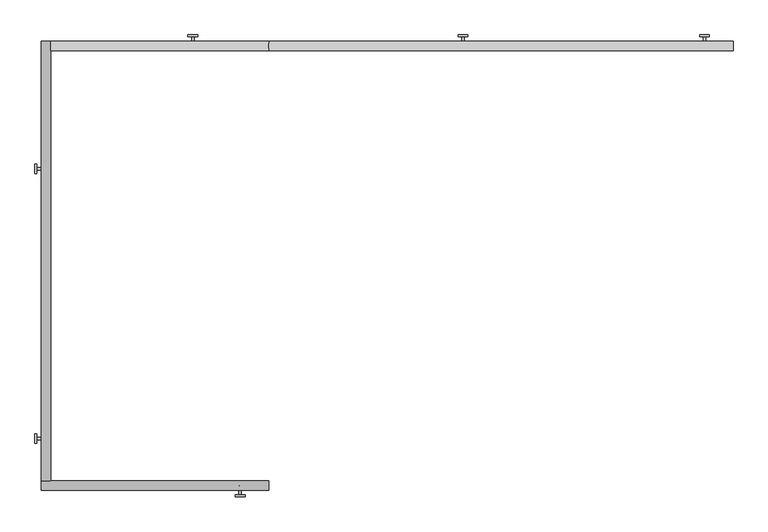
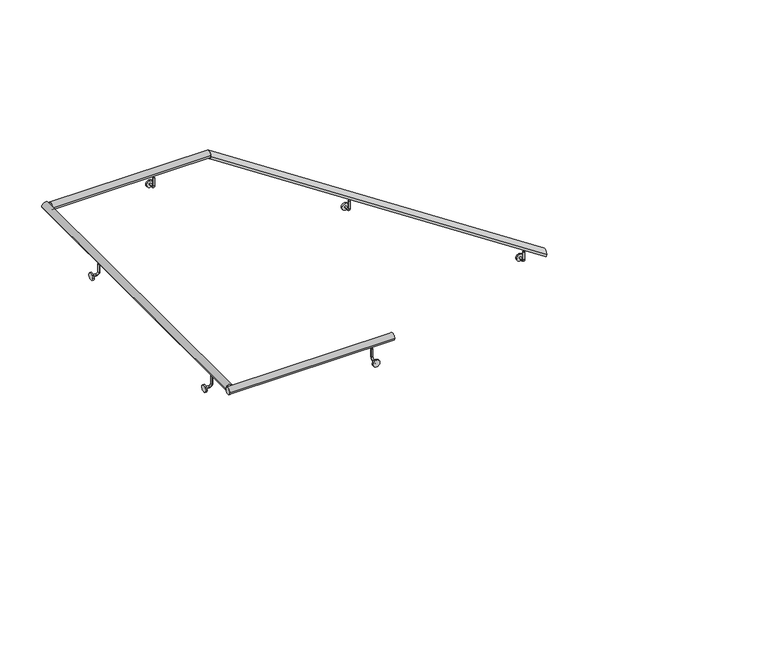
"""IFC4 building model written with IfcOpenShell, lengths in millimetres: railing geometry."""

import ifcopenshell
import ifcopenshell.guid

model = None  # the IFC model being written
_history = None  # IfcOwnerHistory: only IFC2X3 demands one
_inside = {}  # id of a spatial element -> (the spatial element, [elements in it])
_under = {}  # id of a project, library or spatial element -> (it, [spatial elements below it])
_declared = {}  # id of a project -> (the project, [libraries it declares])
_typed = {}  # id of a type object -> (the type object, [elements of that type])
_made_of = {}  # id of a material, layer set ... -> (it, [elements and type objects made of it])


def new_model(schema):
    """Start an empty IFC model of exactly this schema.

    Asked for "IFC4X3", IfcOpenShell would pick the latest addendum, in which some entities
    have other attributes; the version numbers below select the first issue.
    IFC2X3 requires an IfcOwnerHistory on every rooted entity: one is made here for all.
    """
    global model, _history
    if schema == "IFC4X3":
        model = ifcopenshell.file(schema_version=(4, 3, 0, 0))
    else:
        model = ifcopenshell.file(schema=schema)
    _inside.clear()
    _under.clear()
    _declared.clear()
    _typed.clear()
    _made_of.clear()
    _history = None
    if model.schema == "IFC2X3":
        org = make("IfcOrganization", Name="unknown")
        user = make(
            "IfcPersonAndOrganization",
            ThePerson=make("IfcPerson", FamilyName="unknown"),
            TheOrganization=org,
        )
        app = make(
            "IfcApplication",
            ApplicationDeveloper=org,
            Version="unknown",
            ApplicationFullName="unknown",
            ApplicationIdentifier="unknown",
        )
        _history = make(
            "IfcOwnerHistory",
            OwningUser=user,
            OwningApplication=app,
            ChangeAction="ADDED",
            CreationDate=0,
        )
    return model


def make(cls, **values):
    """One entity of the class cls with the attributes given. An attribute that is None is left unset."""
    return model.create_entity(
        cls, **{name: value for name, value in values.items() if value is not None}
    )


def rooted(cls, **values):
    """An entity with a GlobalId (a new one), such as an element, a storey or a relation."""
    return make(cls, GlobalId=ifcopenshell.guid.new(), OwnerHistory=_history, **values)


def si_unit(unit_type, name, prefix=None):
    """IfcSIUnit, for example si_unit("LENGTHUNIT", "METRE", prefix="MILLI")."""
    return make("IfcSIUnit", UnitType=unit_type, Prefix=prefix, Name=name)


def assignment(units):
    """IfcUnitAssignment: the units of a project."""
    return None if units is None else make("IfcUnitAssignment", Units=units)


def point(xyz):
    """IfcCartesianPoint."""
    return None if xyz is None else make("IfcCartesianPoint", Coordinates=xyz)


def direction(xyz):
    """IfcDirection."""
    return None if xyz is None else make("IfcDirection", DirectionRatios=xyz)


def frame(location, z_axis=None, x_axis=None):
    """IfcAxis2Placement3D, a coordinate frame: its origin and axes. An axis left out is left unset."""
    return make(
        "IfcAxis2Placement3D",
        Location=point(location),
        Axis=direction(z_axis),
        RefDirection=direction(x_axis),
    )


def frame_2d(location, x_axis=None):
    """IfcAxis2Placement2D, a coordinate frame in the plane: its origin and x axis."""
    return make(
        "IfcAxis2Placement2D", Location=point(location), RefDirection=direction(x_axis)
    )


def origin():
    """The frame at (0, 0, 0) with its axes left unset."""
    return frame((0.0, 0.0, 0.0))


def place(relative_to, where):
    """IfcLocalPlacement: puts the frame where relative to a parent placement (None: the world)."""
    return make(
        "IfcLocalPlacement", PlacementRelTo=relative_to, RelativePlacement=where
    )


def context(
    kind, dimensions, precision=None, world=None, true_north=None, identifier=None
):
    """IfcGeometricRepresentationContext, for example the 3D "Model" context."""
    return make(
        "IfcGeometricRepresentationContext",
        ContextIdentifier=identifier,
        ContextType=kind,
        CoordinateSpaceDimension=dimensions,
        Precision=precision,
        WorldCoordinateSystem=world,
        TrueNorth=true_north,
    )


def project(units=None, contexts=None):
    """IfcProject with its units and contexts."""
    return rooted(
        "IfcProject",
        Name="project",
        RepresentationContexts=contexts,
        UnitsInContext=assignment(units),
    )


def spatial(cls, under=None, at=None, **own):
    """A site, building, storey or space (cls), placed at a placement, below another one or the project."""
    s = rooted(cls, ObjectPlacement=at, **own)
    if under is not None:
        _under.setdefault(under.id(), (under, []))[1].append(s)
    return s


def circle_curve(where, radius):
    """IfcCircle in the frame where."""
    return make("IfcCircle", Position=where, Radius=radius)


def ellipse_curve(where, semi_axis1, semi_axis2):
    """IfcEllipse in the frame where."""
    return make(
        "IfcEllipse", Position=where, SemiAxis1=semi_axis1, SemiAxis2=semi_axis2
    )


def trimmed(basis, trim1, trim2, sense, master):
    """IfcTrimmedCurve: the piece of a basis curve between two trims."""
    return make(
        "IfcTrimmedCurve",
        BasisCurve=basis,
        Trim1=trim1,
        Trim2=trim2,
        SenseAgreement=sense,
        MasterRepresentation=master,
    )


def segment(curve, same_sense, transition):
    """IfcCompositeCurveSegment."""
    return make(
        "IfcCompositeCurveSegment",
        Transition=transition,
        SameSense=same_sense,
        ParentCurve=curve,
    )


def composite_curve(segments, self_intersect=None):
    """IfcCompositeCurve: segments joined end to end."""
    return make("IfcCompositeCurve", Segments=segments, SelfIntersect=self_intersect)


def outline(outer, holes=None, kind="AREA"):
    """IfcArbitraryClosedProfileDef: a profile drawn as a closed curve; with holes, ...WithVoids."""
    if holes is None:
        return make("IfcArbitraryClosedProfileDef", ProfileType=kind, OuterCurve=outer)
    return make(
        "IfcArbitraryProfileDefWithVoids",
        ProfileType=kind,
        OuterCurve=outer,
        InnerCurves=holes,
    )


def extrude(swept, where, along, depth):
    """IfcExtrudedAreaSolid: the profile swept, set in the frame where, extruded along a direction by depth."""
    return make(
        "IfcExtrudedAreaSolid",
        SweptArea=swept,
        Position=where,
        ExtrudedDirection=direction(along),
        Depth=depth,
    )


def shape(context_of_items, identifier, shape_type, items):
    """IfcShapeRepresentation: the items that make up one representation, for example the "Body"."""
    return make(
        "IfcShapeRepresentation",
        ContextOfItems=context_of_items,
        RepresentationIdentifier=identifier,
        RepresentationType=shape_type,
        Items=items,
    )


def source(mapping_origin, context_of_items, identifier, shape_type, items):
    """IfcRepresentationMap: a shape defined once, which mapped items show again and again."""
    return make(
        "IfcRepresentationMap",
        MappingOrigin=mapping_origin,
        MappedRepresentation=shape(context_of_items, identifier, shape_type, items),
    )


def transform(
    local_origin,
    x_axis=None,
    y_axis=None,
    z_axis=None,
    scale=None,
    scale2=None,
    scale3=None,
    uniform=True,
):
    """IfcCartesianTransformationOperator3D, or its non-uniform kind. x_axis, y_axis, z_axis: its Axis1, 2, 3."""
    if uniform:
        return make(
            "IfcCartesianTransformationOperator3D",
            Axis1=direction(x_axis),
            Axis2=direction(y_axis),
            LocalOrigin=point(local_origin),
            Scale=scale,
            Axis3=direction(z_axis),
        )
    return make(
        "IfcCartesianTransformationOperator3DnonUniform",
        Axis1=direction(x_axis),
        Axis2=direction(y_axis),
        LocalOrigin=point(local_origin),
        Scale=scale,
        Axis3=direction(z_axis),
        Scale2=scale2,
        Scale3=scale3,
    )


def mapped(mapping_source, mapping_target):
    """IfcMappedItem: shows the shape of a source again, moved by a transform."""
    return make(
        "IfcMappedItem", MappingSource=mapping_source, MappingTarget=mapping_target
    )


def made_of(thing, what):
    """Note that an element or type object is made of a material, layer set ...; save() writes the relation."""
    if what is not None:
        _made_of.setdefault(what.id(), (what, []))[1].append(thing)
    return thing


def element(
    cls,
    number,
    at=None,
    inside=None,
    cuts=None,
    type_object=None,
    material=None,
    context=None,
    identifier="Body",
    shape_type=None,
    held_by="IfcProductDefinitionShape",
    body=None,
    shapes=None,
    **own,
):
    """One element of the class cls, such as IfcWall. Its Tag is "e" and its number.

    at: its placement. inside: the storey or other place that contains it. cuts: it is an
    opening in that element (IfcRelVoidsElement). A single representation is given by context,
    identifier, shape_type and body (its items); several are given by shapes. held_by: the class
    of the entity that holds the representations. save() writes the other relations.
    """
    e = rooted(cls, Tag="e%d" % number, ObjectPlacement=at, **own)
    if body is not None:
        shapes = [shape(context, identifier, shape_type, body)]
    if shapes is not None:
        e.Representation = make(held_by, Representations=shapes)
    if inside is not None:
        _inside.setdefault(inside.id(), (inside, []))[1].append(e)
    if cuts is not None:
        rooted(
            "IfcRelVoidsElement", RelatingBuildingElement=cuts, RelatedOpeningElement=e
        )
    if type_object is not None:
        _typed.setdefault(type_object.id(), (type_object, []))[1].append(e)
    return made_of(e, material)


def aggregate(whole, parts):
    """IfcRelAggregates: a whole, such as a stair, and the parts it consists of."""
    return rooted("IfcRelAggregates", RelatingObject=whole, RelatedObjects=parts)


def save(model, path):
    """Write the relations noted so far, then the file.

    IfcRelAggregates (storeys below a building ...), IfcRelContainedInSpatialStructure (elements
    in a storey), IfcRelDefinesByType, IfcRelAssociatesMaterial and IfcRelDeclares: one each for
    every whole, place, type object, material and project.
    """
    for whole, parts in _under.values():
        aggregate(whole, parts)
    for where, things in _inside.values():
        rooted(
            "IfcRelContainedInSpatialStructure",
            RelatedElements=things,
            RelatingStructure=where,
        )
    for kind, things in _typed.values():
        rooted("IfcRelDefinesByType", RelatedObjects=things, RelatingType=kind)
    for what, things in _made_of.values():
        rooted("IfcRelAssociatesMaterial", RelatedObjects=things, RelatingMaterial=what)
    for by, libraries in _declared.values():
        rooted("IfcRelDeclares", RelatingContext=by, RelatedDefinitions=libraries)
    model.write(path)


def plane_surface(at):
    """IfcPlane: the flat surface through the origin of the frame at, square to its z axis."""
    return make("IfcPlane", Position=at)


def cylinder_surface(at, radius):
    """IfcCylindricalSurface: all points at the distance radius from the z axis of the frame at."""
    return make("IfcCylindricalSurface", Position=at, Radius=radius)


def revolved_surface(curve, axis_point, axis_direction):
    """IfcSurfaceOfRevolution: the curve turned about the line through axis_point along axis_direction."""
    return make(
        "IfcSurfaceOfRevolution",
        SweptCurve=make("IfcArbitraryOpenProfileDef", ProfileType="CURVE", Curve=curve),
        AxisPosition=make("IfcAxis1Placement", Location=point(axis_point), Axis=direction(axis_direction)),
    )


def advanced_brep(points, edges, surfaces, faces):
    """IfcAdvancedBrep: a solid bounded by faces that lie on surfaces and meet in shared edges.

    An edge is (start, end): straight between two places in points (the first is 0);
    or (start, end, curve); or (start, end, curve, False) where it runs against its curve.
    A face is (place in surfaces, loops), or (place, loops, False) where it looks against
    its surface's normal. A loop lists edges by number (the first is 1), with a minus sign
    where the edge is run from its end to its start. The first loop is the outer one.
    """
    corners = [point(p) for p in points]
    vertices = [make("IfcVertexPoint", VertexGeometry=c) for c in corners]
    made = []
    for start, end, *more in edges:
        made.append(
            make(
                "IfcEdgeCurve",
                EdgeStart=vertices[start],
                EdgeEnd=vertices[end],
                EdgeGeometry=more[0] if more else make("IfcPolyline", Points=[corners[start], corners[end]]),
                SameSense=more[1] if len(more) > 1 else True,
            )
        )
    hull = []
    for where, loops, *sense in faces:
        bounds = []
        for j, loop in enumerate(loops):
            ring = [make("IfcOrientedEdge", EdgeElement=made[abs(k) - 1], Orientation=k > 0) for k in loop]
            bounds.append(
                make(
                    "IfcFaceOuterBound" if j == 0 else "IfcFaceBound",
                    Bound=make("IfcEdgeLoop", EdgeList=ring),
                    Orientation=True,
                )
            )
        hull.append(make("IfcAdvancedFace", Bounds=bounds, FaceSurface=surfaces[where], SameSense=sense[0] if sense else True))
    return make("IfcAdvancedBrep", Outer=make("IfcClosedShell", CfsFaces=hull))


def railing_2f2e9fd8(model_context):
    return source(origin(), model_context, "Body", "SolidModel", [
        advanced_brep(
        [(-47841.1127262, 17739.1574868, 1147.8451634), (-47841.1127262, 17789.1574868, 1147.8451634), (-50271.1127262, 17739.1574868, 2747.8451634), (-50271.1127262, 17789.1574868, 2747.8451634)],
        [
            (0, 1, ellipse_curve(frame((-47841.1127262, 17764.1574868, 1147.8451634), z_axis=(1.0, 0.0, 0.0), x_axis=(0.0, 0.0, -1.0)), 29.9326144, 25.0)),
            (1, 0, ellipse_curve(frame((-47841.1127262, 17764.1574868, 1147.8451634), z_axis=(1.0, 0.0, 0.0), x_axis=(0.0, 0.0, -1.0)), 29.9326144, 25.0)),
            (2, 3, ellipse_curve(frame((-50271.1127262, 17764.1574868, 2747.8451634), z_axis=(-1.0, 0.0, 0.0), x_axis=(0.0, 0.0, -1.0)), 29.9326144, 25.0)),
            (3, 2, ellipse_curve(frame((-50271.1127262, 17764.1574868, 2747.8451634), z_axis=(-1.0, 0.0, 0.0), x_axis=(0.0, 0.0, -1.0)), 29.9326144, 25.0)),
            (0, 2),
            (3, 1),
        ],
        [
            plane_surface(frame((-47841.1127262, 17764.1574868, 1177.7777778), z_axis=(1.0, 0.0, 0.0), x_axis=(0.0, -1.0, 0.0))),
            plane_surface(frame((-50271.1127262, 17764.1574868, 2777.7777778), z_axis=(-1.0, 0.0, 0.0), x_axis=(0.0, -1.0, 0.0))),
            cylinder_surface(frame((-47854.8610286, 17764.1574868, 1156.8975435), z_axis=(0.8352093694289686, 0.0, -0.5499320950972626), x_axis=(0.0, 1.0, 0.0)), 25.0),
        ],
        [
            (0, [[1, 2]]),
            (1, [[3, 4]]),
            (2, [[-1, 5, -4, 6]]),
            (2, [[-2, -6, -3, -5]]),
        ],
    ),
        advanced_brep(
        [(-50271.1127262, 17739.1574868, 2752.7777778), (-50271.1127262, 17789.1574868, 2752.7777778), (-51413.5127262, 17739.1574868, 2752.7777778), (-51413.5127262, 17789.1574868, 2752.7777778)],
        [
            (0, 1, circle_curve(frame((-50271.1127262, 17764.1574868, 2752.7777778), z_axis=(1.0, 0.0, 0.0), x_axis=(0.0, 1.0, 0.0)), 25.0)),
            (1, 0, circle_curve(frame((-50271.1127262, 17764.1574868, 2752.7777778), z_axis=(1.0, 0.0, 0.0), x_axis=(0.0, 1.0, 0.0)), 25.0)),
            (2, 3, circle_curve(frame((-51413.5127262, 17764.1574868, 2752.7777778), z_axis=(-1.0, 0.0, 0.0), x_axis=(0.0, 1.0, 0.0)), 25.0)),
            (3, 2, circle_curve(frame((-51413.5127262, 17764.1574868, 2752.7777778), z_axis=(-1.0, 0.0, 0.0), x_axis=(0.0, 1.0, 0.0)), 25.0)),
            (0, 2),
            (3, 1),
        ],
        [
            plane_surface(frame((-50271.1127262, 17764.1574868, 2777.7777778), z_axis=(1.0, 0.0, 0.0), x_axis=(0.0, -1.0, 0.0))),
            plane_surface(frame((-51413.5127262, 17764.1574868, 2777.7777778), z_axis=(-1.0, 0.0, 0.0), x_axis=(0.0, -1.0, 0.0))),
            cylinder_surface(frame((-50271.1127262, 17764.1574868, 2752.7777778), z_axis=(1.0, 0.0, 0.0), x_axis=(0.0, 1.0, 0.0)), 25.0),
        ],
        [
            (0, [[1, 2]]),
            (1, [[3, 4]]),
            (2, [[-1, 5, -4, 6]]),
            (2, [[-2, -6, -3, -5]]),
        ],
    ),
        advanced_brep(
        [(-51413.5127262, 17789.1574868, 2752.7777778), (-51463.5127262, 17789.1574868, 2752.7777778), (-51413.5127262, 15484.3587092, 2752.7777778), (-51463.5127262, 15484.3587092, 2752.7777778)],
        [
            (0, 1, circle_curve(frame((-51438.5127262, 17789.1574868, 2752.7777778), z_axis=(0.0, 1.0, 0.0), x_axis=(-1.0, 0.0, 0.0)), 25.0)),
            (1, 0, circle_curve(frame((-51438.5127262, 17789.1574868, 2752.7777778), z_axis=(0.0, 1.0, 0.0), x_axis=(-1.0, 0.0, 0.0)), 25.0)),
            (2, 3, circle_curve(frame((-51438.5127262, 15484.3587092, 2752.7777778), z_axis=(0.0, -1.0, 0.0), x_axis=(-1.0, 0.0, 0.0)), 25.0)),
            (3, 2, circle_curve(frame((-51438.5127262, 15484.3587092, 2752.7777778), z_axis=(0.0, -1.0, 0.0), x_axis=(-1.0, 0.0, 0.0)), 25.0)),
            (0, 2),
            (3, 1),
        ],
        [
            plane_surface(frame((-51438.5127262, 17789.1574868, 2777.7777778), z_axis=(0.0, 1.0, 0.0), x_axis=(0.0, 0.0, -1.0))),
            plane_surface(frame((-51438.5127262, 15484.3587092, 2777.7777778), z_axis=(0.0, -1.0, 0.0), x_axis=(0.0, 0.0, -1.0))),
            cylinder_surface(frame((-51438.5127262, 17789.1574868, 2752.7777778), z_axis=(0.0, 1.0, 0.0), x_axis=(-1.0, 0.0, 0.0)), 25.0),
        ],
        [
            (0, [[1, 2]]),
            (1, [[3, 4]]),
            (2, [[-1, 5, -4, 6]]),
            (2, [[-2, -6, -3, -5]]),
        ],
    ),
        advanced_brep(
        [(-51463.5127262, 15484.3587092, 2752.7777778), (-51463.5127262, 15434.3587092, 2752.7777778), (-50271.1127262, 15484.3587092, 2752.7777778), (-50271.1127262, 15434.3587092, 2752.7777778)],
        [
            (0, 1, circle_curve(frame((-51463.5127262, 15459.3587092, 2752.7777778), z_axis=(-1.0, 0.0, 0.0), x_axis=(0.0, -1.0, 0.0)), 25.0)),
            (1, 0, circle_curve(frame((-51463.5127262, 15459.3587092, 2752.7777778), z_axis=(-1.0, 0.0, 0.0), x_axis=(0.0, -1.0, 0.0)), 25.0)),
            (2, 3, circle_curve(frame((-50271.1127262, 15459.3587092, 2752.7777778), z_axis=(1.0, 0.0, 0.0), x_axis=(0.0, -1.0, 0.0)), 25.0)),
            (3, 2, circle_curve(frame((-50271.1127262, 15459.3587092, 2752.7777778), z_axis=(1.0, 0.0, 0.0), x_axis=(0.0, -1.0, 0.0)), 25.0)),
            (0, 2),
            (3, 1),
        ],
        [
            plane_surface(frame((-51463.5127262, 15459.3587092, 2777.7777778), z_axis=(-1.0, 0.0, 0.0), x_axis=(0.0, 1.0, 0.0))),
            plane_surface(frame((-50271.1127262, 15459.3587092, 2777.7777778), z_axis=(1.0, 0.0, 0.0), x_axis=(0.0, 1.0, 0.0))),
            cylinder_surface(frame((-51463.5127262, 15459.3587092, 2752.7777778), z_axis=(-1.0, 0.0, 0.0), x_axis=(0.0, -1.0, 0.0)), 25.0),
        ],
        [
            (0, [[1, 2]]),
            (1, [[3, 4]]),
            (2, [[-1, 5, -4, 6]]),
            (2, [[-2, -6, -3, -5]]),
        ],
    ),
        advanced_brep(
        [(-51438.5127262, 15712.2284647, 2708.7277778), (-51438.5127262, 15699.5284647, 2708.7277778), (-51438.5127262, 15712.2284647, 2651.5777778), (-51438.5127262, 15699.5284647, 2651.5777778), (-51457.5627262, 15699.5284647, 2632.5277778), (-51457.5627262, 15712.2284647, 2632.5277778), (-51486.1377262, 15712.2284647, 2632.5277778), (-51486.1377262, 15699.5284647, 2632.5277778)],
        [
            (0, 1, circle_curve(frame((-51438.5127262, 15705.8784647, 2708.7277778), z_axis=(0.0, 0.0, 1.0), x_axis=(0.0, -1.0, 0.0)), 6.35)),
            (1, 0, circle_curve(frame((-51438.5127262, 15705.8784647, 2708.7277778), z_axis=(0.0, 0.0, 1.0), x_axis=(0.0, -1.0, 0.0)), 6.35)),
            (0, 2),
            (2, 3, circle_curve(frame((-51438.5127262, 15705.8784647, 2651.5777778), z_axis=(0.0, 0.0, 1.0), x_axis=(0.0, -1.0, 0.0)), 6.35)),
            (3, 1),
            (3, 2, circle_curve(frame((-51438.5127262, 15705.8784647, 2651.5777778), z_axis=(0.0, 0.0, 1.0), x_axis=(0.0, -1.0, 0.0)), 6.35)),
            (4, 3, circle_curve(frame((-51457.5627262, 15699.5284647, 2651.5777778), z_axis=(0.0, -1.0, 0.0), x_axis=(1.0, 0.0, 0.0)), 19.05)),
            (2, 5, circle_curve(frame((-51457.5627262, 15712.2284647, 2651.5777778), z_axis=(0.0, 1.0, 0.0), x_axis=(1.0, 0.0, 0.0)), 19.05)),
            (5, 4, circle_curve(frame((-51457.5627262, 15705.8784647, 2632.5277778), z_axis=(1.0, 0.0, 0.0), x_axis=(0.0, -1.0, 0.0)), 6.35)),
            (4, 5, circle_curve(frame((-51457.5627262, 15705.8784647, 2632.5277778), z_axis=(1.0, 0.0, 0.0), x_axis=(0.0, -1.0, 0.0)), 6.35)),
            (6, 7, circle_curve(frame((-51486.1377262, 15705.8784647, 2632.5277778), z_axis=(-1.0, 0.0, 0.0), x_axis=(0.0, -1.0, 0.0)), 6.35)),
            (7, 6, circle_curve(frame((-51486.1377262, 15705.8784647, 2632.5277778), z_axis=(-1.0, 0.0, 0.0), x_axis=(0.0, -1.0, 0.0)), 6.35)),
            (5, 6),
            (7, 4),
        ],
        [
            plane_surface(frame((-51438.5127262, 15699.5284647, 2708.7277778), z_axis=(0.0, 0.0, 1.0), x_axis=(-1.0, 0.0, 0.0))),
            cylinder_surface(frame((-51438.5127262, 15705.8784647, 2708.7277778), z_axis=(0.0, 0.0, 1.0), x_axis=(0.0, -1.0, 0.0)), 6.35),
            revolved_surface(trimmed(ellipse_curve(frame((-51438.5127262, 15705.8784647, 2651.5777778), z_axis=(0.0, 0.0, 1.0), x_axis=(0.0, -1.0, 0.0)), 6.35, 6.35), [point((-51438.5127262, 15712.2284647, 2651.5777778))], [point((-51438.5127262, 15699.5284647, 2651.5777778))], True, "CARTESIAN"), (-51457.5627262, 15705.8784647, 2651.5777778), (0.0, 1.0, 0.0)),
            revolved_surface(trimmed(ellipse_curve(frame((-51438.5127262, 15705.8784647, 2651.5777778), z_axis=(0.0, 0.0, 1.0), x_axis=(0.0, -1.0, 0.0)), 6.35, 6.35), [point((-51438.5127262, 15699.5284647, 2651.5777778))], [point((-51438.5127262, 15712.2284647, 2651.5777778))], True, "CARTESIAN"), (-51457.5627262, 15705.8784647, 2651.5777778), (0.0, 1.0, 0.0)),
            plane_surface(frame((-51486.1377262, 15705.8784647, 2626.1777778), z_axis=(-1.0, 0.0, 0.0), x_axis=(0.0, -1.0, 0.0))),
            cylinder_surface(frame((-51457.5627262, 15705.8784647, 2632.5277778), z_axis=(1.0, 0.0, 0.0), x_axis=(0.0, -1.0, 0.0)), 6.35),
        ],
        [
            (0, [[1, 2]]),
            (1, [[-1, 3, 4, 5]]),
            (1, [[-2, -5, 6, -3]]),
            (2, [[7, -4, 8, 9]]),
            (3, [[-8, -6, -7, 10]]),
            (4, [[11, 12]]),
            (5, [[-9, 13, -12, 14]]),
            (5, [[-10, -14, -11, -13]]),
        ],
    ),
        extrude(outline(composite_curve([segment(trimmed(circle_curve(frame_2d((15705.8784647, 2632.5277778)), 25.4), [point((15680.4784647, 2632.5277778))], [point((15731.2784647, 2632.5277778))], False, "CARTESIAN"), True, "CONTINUOUS"), segment(trimmed(circle_curve(frame_2d((15705.8784647, 2632.5277778)), 25.4), [point((15731.2784647, 2632.5277778))], [point((15680.4784647, 2632.5277778))], False, "CARTESIAN"), True, "CONTINUOUS")], self_intersect=False)), frame((-51495.6627262, 0.0, 0.0), z_axis=(1.0, 0.0, 0.0), x_axis=(0.0, 1.0, 0.0)), (0.0, 0.0, 1.0), 9.525),
        advanced_brep(
        [(-51438.5127262, 17126.1482202, 2708.7277778), (-51438.5127262, 17113.4482202, 2708.7277778), (-51438.5127262, 17126.1482202, 2651.5777778), (-51438.5127262, 17113.4482202, 2651.5777778), (-51457.5627262, 17113.4482202, 2632.5277778), (-51457.5627262, 17126.1482202, 2632.5277778), (-51486.1377262, 17126.1482202, 2632.5277778), (-51486.1377262, 17113.4482202, 2632.5277778)],
        [
            (0, 1, circle_curve(frame((-51438.5127262, 17119.7982202, 2708.7277778), z_axis=(0.0, 0.0, 1.0), x_axis=(0.0, -1.0, 0.0)), 6.35)),
            (1, 0, circle_curve(frame((-51438.5127262, 17119.7982202, 2708.7277778), z_axis=(0.0, 0.0, 1.0), x_axis=(0.0, -1.0, 0.0)), 6.35)),
            (0, 2),
            (2, 3, circle_curve(frame((-51438.5127262, 17119.7982202, 2651.5777778), z_axis=(0.0, 0.0, 1.0), x_axis=(0.0, -1.0, 0.0)), 6.35)),
            (3, 1),
            (3, 2, circle_curve(frame((-51438.5127262, 17119.7982202, 2651.5777778), z_axis=(0.0, 0.0, 1.0), x_axis=(0.0, -1.0, 0.0)), 6.35)),
            (4, 3, circle_curve(frame((-51457.5627262, 17113.4482202, 2651.5777778), z_axis=(0.0, -1.0, 0.0), x_axis=(1.0, 0.0, 0.0)), 19.05)),
            (2, 5, circle_curve(frame((-51457.5627262, 17126.1482202, 2651.5777778), z_axis=(0.0, 1.0, 0.0), x_axis=(1.0, 0.0, 0.0)), 19.05)),
            (5, 4, circle_curve(frame((-51457.5627262, 17119.7982202, 2632.5277778), z_axis=(1.0, 0.0, 0.0), x_axis=(0.0, -1.0, 0.0)), 6.35)),
            (4, 5, circle_curve(frame((-51457.5627262, 17119.7982202, 2632.5277778), z_axis=(1.0, 0.0, 0.0), x_axis=(0.0, -1.0, 0.0)), 6.35)),
            (6, 7, circle_curve(frame((-51486.1377262, 17119.7982202, 2632.5277778), z_axis=(-1.0, 0.0, 0.0), x_axis=(0.0, -1.0, 0.0)), 6.35)),
            (7, 6, circle_curve(frame((-51486.1377262, 17119.7982202, 2632.5277778), z_axis=(-1.0, 0.0, 0.0), x_axis=(0.0, -1.0, 0.0)), 6.35)),
            (5, 6),
            (7, 4),
        ],
        [
            plane_surface(frame((-51438.5127262, 17113.4482202, 2708.7277778), z_axis=(0.0, 0.0, 1.0), x_axis=(-1.0, 0.0, 0.0))),
            cylinder_surface(frame((-51438.5127262, 17119.7982202, 2708.7277778), z_axis=(0.0, 0.0, 1.0), x_axis=(0.0, -1.0, 0.0)), 6.35),
            revolved_surface(trimmed(ellipse_curve(frame((-51438.5127262, 17119.7982202, 2651.5777778), z_axis=(0.0, 0.0, 1.0), x_axis=(0.0, -1.0, 0.0)), 6.35, 6.35), [point((-51438.5127262, 17126.1482202, 2651.5777778))], [point((-51438.5127262, 17113.4482202, 2651.5777778))], True, "CARTESIAN"), (-51457.5627262, 17119.7982202, 2651.5777778), (0.0, 1.0, 0.0)),
            revolved_surface(trimmed(ellipse_curve(frame((-51438.5127262, 17119.7982202, 2651.5777778), z_axis=(0.0, 0.0, 1.0), x_axis=(0.0, -1.0, 0.0)), 6.35, 6.35), [point((-51438.5127262, 17113.4482202, 2651.5777778))], [point((-51438.5127262, 17126.1482202, 2651.5777778))], True, "CARTESIAN"), (-51457.5627262, 17119.7982202, 2651.5777778), (0.0, 1.0, 0.0)),
            plane_surface(frame((-51486.1377262, 17119.7982202, 2626.1777778), z_axis=(-1.0, 0.0, 0.0), x_axis=(0.0, -1.0, 0.0))),
            cylinder_surface(frame((-51457.5627262, 17119.7982202, 2632.5277778), z_axis=(1.0, 0.0, 0.0), x_axis=(0.0, -1.0, 0.0)), 6.35),
        ],
        [
            (0, [[1, 2]]),
            (1, [[-1, 3, 4, 5]]),
            (1, [[-2, -5, 6, -3]]),
            (2, [[7, -4, 8, 9]]),
            (3, [[-8, -6, -7, 10]]),
            (4, [[11, 12]]),
            (5, [[-9, 13, -12, 14]]),
            (5, [[-10, -14, -11, -13]]),
        ],
    ),
        extrude(outline(composite_curve([segment(trimmed(circle_curve(frame_2d((17119.7982202, 2632.5277778)), 25.4), [point((17094.3982202, 2632.5277778))], [point((17145.1982202, 2632.5277778))], False, "CARTESIAN"), True, "CONTINUOUS"), segment(trimmed(circle_curve(frame_2d((17119.7982202, 2632.5277778)), 25.4), [point((17145.1982202, 2632.5277778))], [point((17094.3982202, 2632.5277778))], False, "CARTESIAN"), True, "CONTINUOUS")], self_intersect=False)), frame((-51495.6627262, 0.0, 0.0), z_axis=(1.0, 0.0, 0.0), x_axis=(0.0, 1.0, 0.0)), (0.0, 0.0, 1.0), 9.525),
        advanced_brep(
        [(-50662.6022373, 17764.1574868, 2708.7277778), (-50675.3022373, 17764.1574868, 2708.7277778), (-50662.6022373, 17764.1574868, 2651.5777778), (-50675.3022373, 17764.1574868, 2651.5777778), (-50675.3022373, 17783.2074868, 2632.5277778), (-50662.6022373, 17783.2074868, 2632.5277778), (-50662.6022373, 17811.7824868, 2632.5277778), (-50675.3022373, 17811.7824868, 2632.5277778)],
        [
            (0, 1, circle_curve(frame((-50668.9522373, 17764.1574868, 2708.7277778), z_axis=(0.0, 0.0, 1.0), x_axis=(-1.0, 0.0, 0.0)), 6.35)),
            (1, 0, circle_curve(frame((-50668.9522373, 17764.1574868, 2708.7277778), z_axis=(0.0, 0.0, 1.0), x_axis=(-1.0, 0.0, 0.0)), 6.35)),
            (0, 2),
            (2, 3, circle_curve(frame((-50668.9522373, 17764.1574868, 2651.5777778), z_axis=(0.0, 0.0, 1.0), x_axis=(-1.0, 0.0, 0.0)), 6.35)),
            (3, 1),
            (3, 2, circle_curve(frame((-50668.9522373, 17764.1574868, 2651.5777778), z_axis=(0.0, 0.0, 1.0), x_axis=(-1.0, 0.0, 0.0)), 6.35)),
            (4, 3, circle_curve(frame((-50675.3022373, 17783.2074868, 2651.5777778), z_axis=(-1.0, 0.0, 0.0), x_axis=(0.0, -1.0, 0.0)), 19.05)),
            (2, 5, circle_curve(frame((-50662.6022373, 17783.2074868, 2651.5777778), z_axis=(1.0, 0.0, 0.0), x_axis=(0.0, -1.0, 0.0)), 19.05)),
            (5, 4, circle_curve(frame((-50668.9522373, 17783.2074868, 2632.5277778), z_axis=(0.0, -1.0, 0.0), x_axis=(-1.0, 0.0, 0.0)), 6.35)),
            (4, 5, circle_curve(frame((-50668.9522373, 17783.2074868, 2632.5277778), z_axis=(0.0, -1.0, 0.0), x_axis=(-1.0, 0.0, 0.0)), 6.35)),
            (6, 7, circle_curve(frame((-50668.9522373, 17811.7824868, 2632.5277778), z_axis=(0.0, 1.0, 0.0), x_axis=(-1.0, 0.0, 0.0)), 6.35)),
            (7, 6, circle_curve(frame((-50668.9522373, 17811.7824868, 2632.5277778), z_axis=(0.0, 1.0, 0.0), x_axis=(-1.0, 0.0, 0.0)), 6.35)),
            (5, 6),
            (7, 4),
        ],
        [
            plane_surface(frame((-50675.3022373, 17764.1574868, 2708.7277778), z_axis=(0.0, 0.0, 1.0), x_axis=(0.0, 1.0, 0.0))),
            cylinder_surface(frame((-50668.9522373, 17764.1574868, 2708.7277778), z_axis=(0.0, 0.0, 1.0), x_axis=(-1.0, 0.0, 0.0)), 6.35),
            revolved_surface(trimmed(ellipse_curve(frame((-50668.9522373, 17764.1574868, 2651.5777778), z_axis=(0.0, 0.0, 1.0), x_axis=(-1.0, 0.0, 0.0)), 6.35, 6.35), [point((-50662.6022373, 17764.1574868, 2651.5777778))], [point((-50675.3022373, 17764.1574868, 2651.5777778))], True, "CARTESIAN"), (-50668.9522373, 17783.2074868, 2651.5777778), (1.0, 0.0, 0.0)),
            revolved_surface(trimmed(ellipse_curve(frame((-50668.9522373, 17764.1574868, 2651.5777778), z_axis=(0.0, 0.0, 1.0), x_axis=(-1.0, 0.0, 0.0)), 6.35, 6.35), [point((-50675.3022373, 17764.1574868, 2651.5777778))], [point((-50662.6022373, 17764.1574868, 2651.5777778))], True, "CARTESIAN"), (-50668.9522373, 17783.2074868, 2651.5777778), (1.0, 0.0, 0.0)),
            plane_surface(frame((-50668.9522373, 17811.7824868, 2626.1777778), z_axis=(0.0, 1.0, 0.0), x_axis=(-1.0, 0.0, 0.0))),
            cylinder_surface(frame((-50668.9522373, 17783.2074868, 2632.5277778), z_axis=(0.0, -1.0, 0.0), x_axis=(-1.0, 0.0, 0.0)), 6.35),
        ],
        [
            (0, [[1, 2]]),
            (1, [[-1, 3, 4, 5]]),
            (1, [[-2, -5, 6, -3]]),
            (2, [[7, -4, 8, 9]]),
            (3, [[-8, -6, -7, 10]]),
            (4, [[11, 12]]),
            (5, [[-9, 13, -12, 14]]),
            (5, [[-10, -14, -11, -13]]),
        ],
    ),
        extrude(outline(composite_curve([segment(trimmed(circle_curve(frame_2d((2632.5277778, -50668.9522373)), 25.4), [point((2632.5277778, -50694.3522373))], [point((2632.5277778, -50643.5522373))], False, "CARTESIAN"), True, "CONTINUOUS"), segment(trimmed(circle_curve(frame_2d((2632.5277778, -50668.9522373)), 25.4), [point((2632.5277778, -50643.5522373))], [point((2632.5277778, -50694.3522373))], False, "CARTESIAN"), True, "CONTINUOUS")], self_intersect=False)), frame((0.0, 17811.7824868, 0.0), z_axis=(0.0, 1.0, 0.0), x_axis=(0.0, 0.0, 1.0)), (0.0, 0.0, 1.0), 9.525),
        advanced_brep(
        [(-49248.6824817, 17764.1574868, 2039.7037485), (-49261.3824817, 17764.1574868, 2039.7037485), (-49248.6824817, 17764.1574868, 1982.5537485), (-49261.3824817, 17764.1574868, 1982.5537485), (-49261.3824817, 17783.2074868, 1963.5037485), (-49248.6824817, 17783.2074868, 1963.5037485), (-49248.6824817, 17811.7824868, 1963.5037485), (-49261.3824817, 17811.7824868, 1963.5037485)],
        [
            (0, 1, circle_curve(frame((-49255.0324817, 17764.1574868, 2039.7037485), z_axis=(0.0, 0.0, 1.0), x_axis=(-1.0, 0.0, 0.0)), 6.35)),
            (1, 0, circle_curve(frame((-49255.0324817, 17764.1574868, 2039.7037485), z_axis=(0.0, 0.0, 1.0), x_axis=(-1.0, 0.0, 0.0)), 6.35)),
            (0, 2),
            (2, 3, circle_curve(frame((-49255.0324817, 17764.1574868, 1982.5537485), z_axis=(0.0, 0.0, 1.0), x_axis=(-1.0, 0.0, 0.0)), 6.35)),
            (3, 1),
            (3, 2, circle_curve(frame((-49255.0324817, 17764.1574868, 1982.5537485), z_axis=(0.0, 0.0, 1.0), x_axis=(-1.0, 0.0, 0.0)), 6.35)),
            (4, 3, circle_curve(frame((-49261.3824817, 17783.2074868, 1982.5537485), z_axis=(-1.0, 0.0, 0.0), x_axis=(0.0, -1.0, 0.0)), 19.05)),
            (2, 5, circle_curve(frame((-49248.6824817, 17783.2074868, 1982.5537485), z_axis=(1.0, 0.0, 0.0), x_axis=(0.0, -1.0, 0.0)), 19.05)),
            (5, 4, circle_curve(frame((-49255.0324817, 17783.2074868, 1963.5037485), z_axis=(0.0, -1.0, 0.0), x_axis=(-1.0, 0.0, 0.0)), 6.35)),
            (4, 5, circle_curve(frame((-49255.0324817, 17783.2074868, 1963.5037485), z_axis=(0.0, -1.0, 0.0), x_axis=(-1.0, 0.0, 0.0)), 6.35)),
            (6, 7, circle_curve(frame((-49255.0324817, 17811.7824868, 1963.5037485), z_axis=(0.0, 1.0, 0.0), x_axis=(-1.0, 0.0, 0.0)), 6.35)),
            (7, 6, circle_curve(frame((-49255.0324817, 17811.7824868, 1963.5037485), z_axis=(0.0, 1.0, 0.0), x_axis=(-1.0, 0.0, 0.0)), 6.35)),
            (5, 6),
            (7, 4),
        ],
        [
            plane_surface(frame((-49261.3824817, 17764.1574868, 2039.7037485), z_axis=(0.0, 0.0, 1.0), x_axis=(0.0, 1.0, 0.0))),
            cylinder_surface(frame((-49255.0324817, 17764.1574868, 2039.7037485), z_axis=(0.0, 0.0, 1.0), x_axis=(-1.0, 0.0, 0.0)), 6.35),
            revolved_surface(trimmed(ellipse_curve(frame((-49255.0324817, 17764.1574868, 1982.5537485), z_axis=(0.0, 0.0, 1.0), x_axis=(-1.0, 0.0, 0.0)), 6.35, 6.35), [point((-49248.6824817, 17764.1574868, 1982.5537485))], [point((-49261.3824817, 17764.1574868, 1982.5537485))], True, "CARTESIAN"), (-49255.0324817, 17783.2074868, 1982.5537485), (1.0, 0.0, 0.0)),
            revolved_surface(trimmed(ellipse_curve(frame((-49255.0324817, 17764.1574868, 1982.5537485), z_axis=(0.0, 0.0, 1.0), x_axis=(-1.0, 0.0, 0.0)), 6.35, 6.35), [point((-49261.3824817, 17764.1574868, 1982.5537485))], [point((-49248.6824817, 17764.1574868, 1982.5537485))], True, "CARTESIAN"), (-49255.0324817, 17783.2074868, 1982.5537485), (1.0, 0.0, 0.0)),
            plane_surface(frame((-49255.0324817, 17811.7824868, 1957.1537485), z_axis=(0.0, 1.0, 0.0), x_axis=(-1.0, 0.0, 0.0))),
            cylinder_surface(frame((-49255.0324817, 17783.2074868, 1963.5037485), z_axis=(0.0, -1.0, 0.0), x_axis=(-1.0, 0.0, 0.0)), 6.35),
        ],
        [
            (0, [[1, 2]]),
            (1, [[-1, 3, 4, 5]]),
            (1, [[-2, -5, 6, -3]]),
            (2, [[7, -4, 8, 9]]),
            (3, [[-8, -6, -7, 10]]),
            (4, [[11, 12]]),
            (5, [[-9, 13, -12, 14]]),
            (5, [[-10, -14, -11, -13]]),
        ],
    ),
        extrude(outline(composite_curve([segment(trimmed(circle_curve(frame_2d((1963.5037485, -49255.0324817)), 25.4), [point((1963.5037485, -49280.4324817))], [point((1963.5037485, -49229.6324817))], False, "CARTESIAN"), True, "CONTINUOUS"), segment(trimmed(circle_curve(frame_2d((1963.5037485, -49255.0324817)), 25.4), [point((1963.5037485, -49229.6324817))], [point((1963.5037485, -49280.4324817))], False, "CARTESIAN"), True, "CONTINUOUS")], self_intersect=False)), frame((0.0, 17811.7824868, 0.0), z_axis=(0.0, 1.0, 0.0), x_axis=(0.0, 0.0, 1.0)), (0.0, 0.0, 1.0), 9.525),
        advanced_brep(
        [(-50427.4627262, 15459.3587092, 2708.7277778), (-50414.7627262, 15459.3587092, 2708.7277778), (-50427.4627262, 15459.3587092, 2651.5777778), (-50414.7627262, 15459.3587092, 2651.5777778), (-50414.7627262, 15440.3087092, 2632.5277778), (-50427.4627262, 15440.3087092, 2632.5277778), (-50427.4627262, 15411.7337092, 2632.5277778), (-50414.7627262, 15411.7337092, 2632.5277778)],
        [
            (0, 1, circle_curve(frame((-50421.1127262, 15459.3587092, 2708.7277778), z_axis=(0.0, 0.0, 1.0), x_axis=(1.0, 0.0, 0.0)), 6.35)),
            (1, 0, circle_curve(frame((-50421.1127262, 15459.3587092, 2708.7277778), z_axis=(0.0, 0.0, 1.0), x_axis=(1.0, 0.0, 0.0)), 6.35)),
            (0, 2),
            (2, 3, circle_curve(frame((-50421.1127262, 15459.3587092, 2651.5777778), z_axis=(0.0, 0.0, 1.0), x_axis=(1.0, 0.0, 0.0)), 6.35)),
            (3, 1),
            (3, 2, circle_curve(frame((-50421.1127262, 15459.3587092, 2651.5777778), z_axis=(0.0, 0.0, 1.0), x_axis=(1.0, 0.0, 0.0)), 6.35)),
            (4, 3, circle_curve(frame((-50414.7627262, 15440.3087092, 2651.5777778), z_axis=(1.0, 0.0, 0.0), x_axis=(0.0, 1.0, 0.0)), 19.05)),
            (2, 5, circle_curve(frame((-50427.4627262, 15440.3087092, 2651.5777778), z_axis=(-1.0, 0.0, 0.0), x_axis=(0.0, 1.0, 0.0)), 19.05)),
            (5, 4, circle_curve(frame((-50421.1127262, 15440.3087092, 2632.5277778), z_axis=(0.0, 1.0, 0.0), x_axis=(1.0, 0.0, 0.0)), 6.35)),
            (4, 5, circle_curve(frame((-50421.1127262, 15440.3087092, 2632.5277778), z_axis=(0.0, 1.0, 0.0), x_axis=(1.0, 0.0, 0.0)), 6.35)),
            (6, 7, circle_curve(frame((-50421.1127262, 15411.7337092, 2632.5277778), z_axis=(0.0, -1.0, 0.0), x_axis=(1.0, 0.0, 0.0)), 6.35)),
            (7, 6, circle_curve(frame((-50421.1127262, 15411.7337092, 2632.5277778), z_axis=(0.0, -1.0, 0.0), x_axis=(1.0, 0.0, 0.0)), 6.35)),
            (5, 6),
            (7, 4),
        ],
        [
            plane_surface(frame((-50414.7627262, 15459.3587092, 2708.7277778), z_axis=(0.0, 0.0, 1.0), x_axis=(0.0, -1.0, 0.0))),
            cylinder_surface(frame((-50421.1127262, 15459.3587092, 2708.7277778), z_axis=(0.0, 0.0, 1.0), x_axis=(1.0, 0.0, 0.0)), 6.35),
            revolved_surface(trimmed(ellipse_curve(frame((-50421.1127262, 15459.3587092, 2651.5777778), z_axis=(0.0, 0.0, 1.0), x_axis=(1.0, 0.0, 0.0)), 6.35, 6.35), [point((-50427.4627262, 15459.3587092, 2651.5777778))], [point((-50414.7627262, 15459.3587092, 2651.5777778))], True, "CARTESIAN"), (-50421.1127262, 15440.3087092, 2651.5777778), (-1.0, 0.0, 0.0)),
            revolved_surface(trimmed(ellipse_curve(frame((-50421.1127262, 15459.3587092, 2651.5777778), z_axis=(0.0, 0.0, 1.0), x_axis=(1.0, 0.0, 0.0)), 6.35, 6.35), [point((-50414.7627262, 15459.3587092, 2651.5777778))], [point((-50427.4627262, 15459.3587092, 2651.5777778))], True, "CARTESIAN"), (-50421.1127262, 15440.3087092, 2651.5777778), (-1.0, 0.0, 0.0)),
            plane_surface(frame((-50421.1127262, 15411.7337092, 2626.1777778), z_axis=(0.0, -1.0, 0.0), x_axis=(1.0, 0.0, 0.0))),
            cylinder_surface(frame((-50421.1127262, 15440.3087092, 2632.5277778), z_axis=(0.0, 1.0, 0.0), x_axis=(1.0, 0.0, 0.0)), 6.35),
        ],
        [
            (0, [[1, 2]]),
            (1, [[-1, 3, 4, 5]]),
            (1, [[-2, -5, 6, -3]]),
            (2, [[7, -4, 8, 9]]),
            (3, [[-8, -6, -7, 10]]),
            (4, [[11, 12]]),
            (5, [[-9, 13, -12, 14]]),
            (5, [[-10, -14, -11, -13]]),
        ],
    ),
        extrude(outline(composite_curve([segment(trimmed(circle_curve(frame_2d((2632.5277778, -50421.1127262)), 25.4), [point((2632.5277778, -50395.7127262))], [point((2632.5277778, -50446.5127262))], False, "CARTESIAN"), True, "CONTINUOUS"), segment(trimmed(circle_curve(frame_2d((2632.5277778, -50421.1127262)), 25.4), [point((2632.5277778, -50446.5127262))], [point((2632.5277778, -50395.7127262))], False, "CARTESIAN"), True, "CONTINUOUS")], self_intersect=False)), frame((0.0, 15402.2087092, 0.0), z_axis=(0.0, 1.0, 0.0), x_axis=(0.0, 0.0, 1.0)), (0.0, 0.0, 1.0), 9.525),
        advanced_brep(
        [(-47984.7627262, 17764.1574868, 1207.4932099), (-47997.4627262, 17764.1574868, 1207.4932099), (-47984.7627262, 17764.1574868, 1150.3432099), (-47997.4627262, 17764.1574868, 1150.3432099), (-47997.4627262, 17783.2074868, 1131.2932099), (-47984.7627262, 17783.2074868, 1131.2932099), (-47984.7627262, 17811.7824868, 1131.2932099), (-47997.4627262, 17811.7824868, 1131.2932099)],
        [
            (0, 1, circle_curve(frame((-47991.1127262, 17764.1574868, 1207.4932099), z_axis=(0.0, 0.0, 1.0), x_axis=(-1.0, 0.0, 0.0)), 6.35)),
            (1, 0, circle_curve(frame((-47991.1127262, 17764.1574868, 1207.4932099), z_axis=(0.0, 0.0, 1.0), x_axis=(-1.0, 0.0, 0.0)), 6.35)),
            (0, 2),
            (2, 3, circle_curve(frame((-47991.1127262, 17764.1574868, 1150.3432099), z_axis=(0.0, 0.0, 1.0), x_axis=(-1.0, 0.0, 0.0)), 6.35)),
            (3, 1),
            (3, 2, circle_curve(frame((-47991.1127262, 17764.1574868, 1150.3432099), z_axis=(0.0, 0.0, 1.0), x_axis=(-1.0, 0.0, 0.0)), 6.35)),
            (4, 3, circle_curve(frame((-47997.4627262, 17783.2074868, 1150.3432099), z_axis=(-1.0, 0.0, 0.0), x_axis=(0.0, -1.0, 0.0)), 19.05)),
            (2, 5, circle_curve(frame((-47984.7627262, 17783.2074868, 1150.3432099), z_axis=(1.0, 0.0, 0.0), x_axis=(0.0, -1.0, 0.0)), 19.05)),
            (5, 4, circle_curve(frame((-47991.1127262, 17783.2074868, 1131.2932099), z_axis=(0.0, -1.0, 0.0), x_axis=(-1.0, 0.0, 0.0)), 6.35)),
            (4, 5, circle_curve(frame((-47991.1127262, 17783.2074868, 1131.2932099), z_axis=(0.0, -1.0, 0.0), x_axis=(-1.0, 0.0, 0.0)), 6.35)),
            (6, 7, circle_curve(frame((-47991.1127262, 17811.7824868, 1131.2932099), z_axis=(0.0, 1.0, 0.0), x_axis=(-1.0, 0.0, 0.0)), 6.35)),
            (7, 6, circle_curve(frame((-47991.1127262, 17811.7824868, 1131.2932099), z_axis=(0.0, 1.0, 0.0), x_axis=(-1.0, 0.0, 0.0)), 6.35)),
            (5, 6),
            (7, 4),
        ],
        [
            plane_surface(frame((-47997.4627262, 17764.1574868, 1207.4932099), z_axis=(0.0, 0.0, 1.0), x_axis=(0.0, 1.0, 0.0))),
            cylinder_surface(frame((-47991.1127262, 17764.1574868, 1207.4932099), z_axis=(0.0, 0.0, 1.0), x_axis=(-1.0, 0.0, 0.0)), 6.35),
            revolved_surface(trimmed(ellipse_curve(frame((-47991.1127262, 17764.1574868, 1150.3432099), z_axis=(0.0, 0.0, 1.0), x_axis=(-1.0, 0.0, 0.0)), 6.35, 6.35), [point((-47984.7627262, 17764.1574868, 1150.3432099))], [point((-47997.4627262, 17764.1574868, 1150.3432099))], True, "CARTESIAN"), (-47991.1127262, 17783.2074868, 1150.3432099), (1.0, 0.0, 0.0)),
            revolved_surface(trimmed(ellipse_curve(frame((-47991.1127262, 17764.1574868, 1150.3432099), z_axis=(0.0, 0.0, 1.0), x_axis=(-1.0, 0.0, 0.0)), 6.35, 6.35), [point((-47997.4627262, 17764.1574868, 1150.3432099))], [point((-47984.7627262, 17764.1574868, 1150.3432099))], True, "CARTESIAN"), (-47991.1127262, 17783.2074868, 1150.3432099), (1.0, 0.0, 0.0)),
            plane_surface(frame((-47991.1127262, 17811.7824868, 1124.9432099), z_axis=(0.0, 1.0, 0.0), x_axis=(-1.0, 0.0, 0.0))),
            cylinder_surface(frame((-47991.1127262, 17783.2074868, 1131.2932099), z_axis=(0.0, -1.0, 0.0), x_axis=(-1.0, 0.0, 0.0)), 6.35),
        ],
        [
            (0, [[1, 2]]),
            (1, [[-1, 3, 4, 5]]),
            (1, [[-2, -5, 6, -3]]),
            (2, [[7, -4, 8, 9]]),
            (3, [[-8, -6, -7, 10]]),
            (4, [[11, 12]]),
            (5, [[-9, 13, -12, 14]]),
            (5, [[-10, -14, -11, -13]]),
        ],
    ),
        extrude(outline(composite_curve([segment(trimmed(circle_curve(frame_2d((1131.2932099, -47991.1127262)), 25.4), [point((1131.2932099, -48016.5127262))], [point((1131.2932099, -47965.7127262))], False, "CARTESIAN"), True, "CONTINUOUS"), segment(trimmed(circle_curve(frame_2d((1131.2932099, -47991.1127262)), 25.4), [point((1131.2932099, -47965.7127262))], [point((1131.2932099, -48016.5127262))], False, "CARTESIAN"), True, "CONTINUOUS")], self_intersect=False)), frame((0.0, 17811.7824868, 0.0), z_axis=(0.0, 1.0, 0.0), x_axis=(0.0, 0.0, 1.0)), (0.0, 0.0, 1.0), 9.525),
    ])


if __name__ == "__main__":
    model = new_model("IFC4")
    model_context = context("Model", 3, world=origin())
    ifc_project = project(units=[si_unit("LENGTHUNIT", "METRE", prefix="MILLI")], contexts=[model_context])
    site = spatial("IfcSite", under=ifc_project)
    building = spatial("IfcBuilding", under=site)
    placement = place(None, origin())
    railing_shape = railing_2f2e9fd8(model_context)
    element("IfcRailing", 1, at=placement, inside=building, context=model_context, shape_type="MappedRepresentation", body=[
        mapped(railing_shape, transform((0.0, 0.0, 0.0), x_axis=(1.0, 0.0, 0.0), y_axis=(0.0, 1.0, 0.0), z_axis=(0.0, 0.0, 1.0))),
    ])
    save(model, "model.ifc")

# Revit data of these elements
# Project information
#   Projekt-Nummer = "Hier die Projektnummer eintragen!"
#   IfcSite GUID = "3DdyCULLv3kQRx$MQ8PThJ"
#   IfcBuilding GUID = "3DdyCULLv3kQRx$MQ8PThG"
#   IfcProject GUID = "3DdyCULLv3kQRx$MQ8PThH"
#   Classification.Facility.Number = "Co_20_15_58"
#   Classification.Facility.Description = "Office complexes"
#   Project Status = "Projektstatus"
#   Project Address = "Geben Sie die Adresse hier ein"
